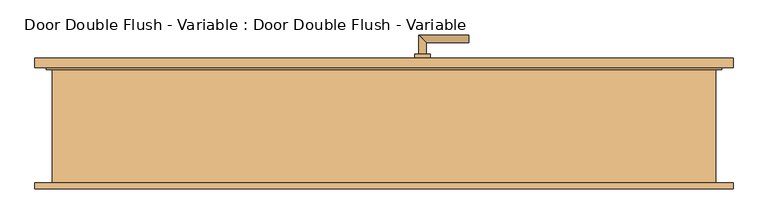
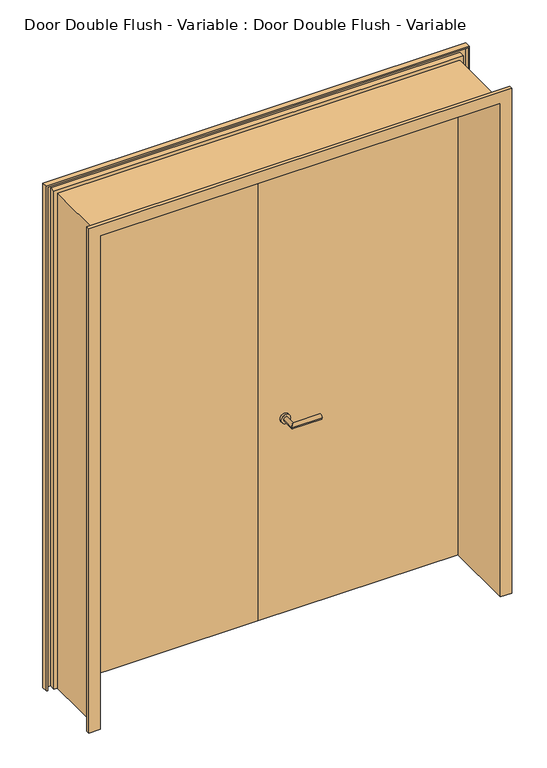
"""IFC4 building model written with IfcOpenShell, lengths in millimetres: door geometry, Door Double Flush - Variable : Door Double Flush - Variable."""

import ifcopenshell
import ifcopenshell.guid

model = None  # the IFC model being written
_history = None  # IfcOwnerHistory: only IFC2X3 demands one
_inside = {}  # id of a spatial element -> (the spatial element, [elements in it])
_under = {}  # id of a project, library or spatial element -> (it, [spatial elements below it])
_declared = {}  # id of a project -> (the project, [libraries it declares])
_typed = {}  # id of a type object -> (the type object, [elements of that type])
_made_of = {}  # id of a material, layer set ... -> (it, [elements and type objects made of it])


def new_model(schema):
    """Start an empty IFC model of exactly this schema.

    Asked for "IFC4X3", IfcOpenShell would pick the latest addendum, in which some entities
    have other attributes; the version numbers below select the first issue.
    IFC2X3 requires an IfcOwnerHistory on every rooted entity: one is made here for all.
    """
    global model, _history
    if schema == "IFC4X3":
        model = ifcopenshell.file(schema_version=(4, 3, 0, 0))
    else:
        model = ifcopenshell.file(schema=schema)
    _inside.clear()
    _under.clear()
    _declared.clear()
    _typed.clear()
    _made_of.clear()
    _history = None
    if model.schema == "IFC2X3":
        org = make("IfcOrganization", Name="unknown")
        user = make(
            "IfcPersonAndOrganization",
            ThePerson=make("IfcPerson", FamilyName="unknown"),
            TheOrganization=org,
        )
        app = make(
            "IfcApplication",
            ApplicationDeveloper=org,
            Version="unknown",
            ApplicationFullName="unknown",
            ApplicationIdentifier="unknown",
        )
        _history = make(
            "IfcOwnerHistory",
            OwningUser=user,
            OwningApplication=app,
            ChangeAction="ADDED",
            CreationDate=0,
        )
    return model


def make(cls, **values):
    """One entity of the class cls with the attributes given. An attribute that is None is left unset."""
    return model.create_entity(
        cls, **{name: value for name, value in values.items() if value is not None}
    )


def rooted(cls, **values):
    """An entity with a GlobalId (a new one), such as an element, a storey or a relation."""
    return make(cls, GlobalId=ifcopenshell.guid.new(), OwnerHistory=_history, **values)


def si_unit(unit_type, name, prefix=None):
    """IfcSIUnit, for example si_unit("LENGTHUNIT", "METRE", prefix="MILLI")."""
    return make("IfcSIUnit", UnitType=unit_type, Prefix=prefix, Name=name)


def assignment(units):
    """IfcUnitAssignment: the units of a project."""
    return None if units is None else make("IfcUnitAssignment", Units=units)


def point(xyz):
    """IfcCartesianPoint."""
    return None if xyz is None else make("IfcCartesianPoint", Coordinates=xyz)


def direction(xyz):
    """IfcDirection."""
    return None if xyz is None else make("IfcDirection", DirectionRatios=xyz)


def frame(location, z_axis=None, x_axis=None):
    """IfcAxis2Placement3D, a coordinate frame: its origin and axes. An axis left out is left unset."""
    return make(
        "IfcAxis2Placement3D",
        Location=point(location),
        Axis=direction(z_axis),
        RefDirection=direction(x_axis),
    )


def frame_2d(location, x_axis=None):
    """IfcAxis2Placement2D, a coordinate frame in the plane: its origin and x axis."""
    return make(
        "IfcAxis2Placement2D", Location=point(location), RefDirection=direction(x_axis)
    )


def origin():
    """The frame at (0, 0, 0) with its axes left unset."""
    return frame((0.0, 0.0, 0.0))


def place(relative_to, where):
    """IfcLocalPlacement: puts the frame where relative to a parent placement (None: the world)."""
    return make(
        "IfcLocalPlacement", PlacementRelTo=relative_to, RelativePlacement=where
    )


def context(
    kind, dimensions, precision=None, world=None, true_north=None, identifier=None
):
    """IfcGeometricRepresentationContext, for example the 3D "Model" context."""
    return make(
        "IfcGeometricRepresentationContext",
        ContextIdentifier=identifier,
        ContextType=kind,
        CoordinateSpaceDimension=dimensions,
        Precision=precision,
        WorldCoordinateSystem=world,
        TrueNorth=true_north,
    )


def project(units=None, contexts=None):
    """IfcProject with its units and contexts."""
    return rooted(
        "IfcProject",
        Name="project",
        RepresentationContexts=contexts,
        UnitsInContext=assignment(units),
    )


def spatial(cls, under=None, at=None, **own):
    """A site, building, storey or space (cls), placed at a placement, below another one or the project."""
    s = rooted(cls, ObjectPlacement=at, **own)
    if under is not None:
        _under.setdefault(under.id(), (under, []))[1].append(s)
    return s


def polyline(points):
    """IfcPolyline through the points."""
    return make("IfcPolyline", Points=[point(p) for p in points])


def circle_curve(where, radius):
    """IfcCircle in the frame where."""
    return make("IfcCircle", Position=where, Radius=radius)


def ellipse_curve(where, semi_axis1, semi_axis2):
    """IfcEllipse in the frame where."""
    return make(
        "IfcEllipse", Position=where, SemiAxis1=semi_axis1, SemiAxis2=semi_axis2
    )


def trimmed(basis, trim1, trim2, sense, master):
    """IfcTrimmedCurve: the piece of a basis curve between two trims."""
    return make(
        "IfcTrimmedCurve",
        BasisCurve=basis,
        Trim1=trim1,
        Trim2=trim2,
        SenseAgreement=sense,
        MasterRepresentation=master,
    )


def segment(curve, same_sense, transition):
    """IfcCompositeCurveSegment."""
    return make(
        "IfcCompositeCurveSegment",
        Transition=transition,
        SameSense=same_sense,
        ParentCurve=curve,
    )


def composite_curve(segments, self_intersect=None):
    """IfcCompositeCurve: segments joined end to end."""
    return make("IfcCompositeCurve", Segments=segments, SelfIntersect=self_intersect)


def outline(outer, holes=None, kind="AREA"):
    """IfcArbitraryClosedProfileDef: a profile drawn as a closed curve; with holes, ...WithVoids."""
    if holes is None:
        return make("IfcArbitraryClosedProfileDef", ProfileType=kind, OuterCurve=outer)
    return make(
        "IfcArbitraryProfileDefWithVoids",
        ProfileType=kind,
        OuterCurve=outer,
        InnerCurves=holes,
    )


def extrude(swept, where, along, depth):
    """IfcExtrudedAreaSolid: the profile swept, set in the frame where, extruded along a direction by depth."""
    return make(
        "IfcExtrudedAreaSolid",
        SweptArea=swept,
        Position=where,
        ExtrudedDirection=direction(along),
        Depth=depth,
    )


def faces_of(points, faces, orient=None, outer=None):
    """IfcFace entities. A face is a list of loops; a loop is a list of indices into points, from 0.

    orient and outer hold one flag for each loop. By default every Orientation is true, the
    first loop of a face is its IfcFaceOuterBound and the others are IfcFaceBound.
    """
    made = []
    for i, loops in enumerate(faces):
        bounds = []
        for j, loop in enumerate(loops):
            is_outer = j == 0 if outer is None else outer[i][j]
            bounds.append(
                make(
                    "IfcFaceOuterBound" if is_outer else "IfcFaceBound",
                    Bound=make("IfcPolyLoop", Polygon=[points[k] for k in loop]),
                    Orientation=True if orient is None else orient[i][j],
                )
            )
        made.append(make("IfcFace", Bounds=bounds))
    return made


def faceted_brep(points, faces, orient=None, outer=None, voids=None):
    """IfcFacetedBrep: a solid bounded by flat faces; with voids (closed shells), ...WithVoids."""
    shared = [point(p) for p in points]
    hull = make("IfcClosedShell", CfsFaces=faces_of(shared, faces, orient, outer))
    if voids is None:
        return make("IfcFacetedBrep", Outer=hull)
    return make(
        "IfcFacetedBrepWithVoids",
        Outer=hull,
        Voids=[
            make(cls, CfsFaces=faces_of(shared, fs, o, b)) for cls, fs, o, b in voids
        ],
    )


def shape(context_of_items, identifier, shape_type, items):
    """IfcShapeRepresentation: the items that make up one representation, for example the "Body"."""
    return make(
        "IfcShapeRepresentation",
        ContextOfItems=context_of_items,
        RepresentationIdentifier=identifier,
        RepresentationType=shape_type,
        Items=items,
    )


def source(mapping_origin, context_of_items, identifier, shape_type, items):
    """IfcRepresentationMap: a shape defined once, which mapped items show again and again."""
    return make(
        "IfcRepresentationMap",
        MappingOrigin=mapping_origin,
        MappedRepresentation=shape(context_of_items, identifier, shape_type, items),
    )


def transform(
    local_origin,
    x_axis=None,
    y_axis=None,
    z_axis=None,
    scale=None,
    scale2=None,
    scale3=None,
    uniform=True,
):
    """IfcCartesianTransformationOperator3D, or its non-uniform kind. x_axis, y_axis, z_axis: its Axis1, 2, 3."""
    if uniform:
        return make(
            "IfcCartesianTransformationOperator3D",
            Axis1=direction(x_axis),
            Axis2=direction(y_axis),
            LocalOrigin=point(local_origin),
            Scale=scale,
            Axis3=direction(z_axis),
        )
    return make(
        "IfcCartesianTransformationOperator3DnonUniform",
        Axis1=direction(x_axis),
        Axis2=direction(y_axis),
        LocalOrigin=point(local_origin),
        Scale=scale,
        Axis3=direction(z_axis),
        Scale2=scale2,
        Scale3=scale3,
    )


def mapped(mapping_source, mapping_target):
    """IfcMappedItem: shows the shape of a source again, moved by a transform."""
    return make(
        "IfcMappedItem", MappingSource=mapping_source, MappingTarget=mapping_target
    )


def made_of(thing, what):
    """Note that an element or type object is made of a material, layer set ...; save() writes the relation."""
    if what is not None:
        _made_of.setdefault(what.id(), (what, []))[1].append(thing)
    return thing


def element(
    cls,
    number,
    at=None,
    inside=None,
    cuts=None,
    type_object=None,
    material=None,
    context=None,
    identifier="Body",
    shape_type=None,
    held_by="IfcProductDefinitionShape",
    body=None,
    shapes=None,
    **own,
):
    """One element of the class cls, such as IfcWall. Its Tag is "e" and its number.

    at: its placement. inside: the storey or other place that contains it. cuts: it is an
    opening in that element (IfcRelVoidsElement). A single representation is given by context,
    identifier, shape_type and body (its items); several are given by shapes. held_by: the class
    of the entity that holds the representations. save() writes the other relations.
    """
    e = rooted(cls, Tag="e%d" % number, ObjectPlacement=at, **own)
    if body is not None:
        shapes = [shape(context, identifier, shape_type, body)]
    if shapes is not None:
        e.Representation = make(held_by, Representations=shapes)
    if inside is not None:
        _inside.setdefault(inside.id(), (inside, []))[1].append(e)
    if cuts is not None:
        rooted(
            "IfcRelVoidsElement", RelatingBuildingElement=cuts, RelatedOpeningElement=e
        )
    if type_object is not None:
        _typed.setdefault(type_object.id(), (type_object, []))[1].append(e)
    return made_of(e, material)


def aggregate(whole, parts):
    """IfcRelAggregates: a whole, such as a stair, and the parts it consists of."""
    return rooted("IfcRelAggregates", RelatingObject=whole, RelatedObjects=parts)


def save(model, path):
    """Write the relations noted so far, then the file.

    IfcRelAggregates (storeys below a building ...), IfcRelContainedInSpatialStructure (elements
    in a storey), IfcRelDefinesByType, IfcRelAssociatesMaterial and IfcRelDeclares: one each for
    every whole, place, type object, material and project.
    """
    for whole, parts in _under.values():
        aggregate(whole, parts)
    for where, things in _inside.values():
        rooted(
            "IfcRelContainedInSpatialStructure",
            RelatedElements=things,
            RelatingStructure=where,
        )
    for kind, things in _typed.values():
        rooted("IfcRelDefinesByType", RelatedObjects=things, RelatingType=kind)
    for what, things in _made_of.values():
        rooted("IfcRelAssociatesMaterial", RelatedObjects=things, RelatingMaterial=what)
    for by, libraries in _declared.values():
        rooted("IfcRelDeclares", RelatingContext=by, RelatedDefinitions=libraries)
    model.write(path)


def plane_surface(at):
    """IfcPlane: the flat surface through the origin of the frame at, square to its z axis."""
    return make("IfcPlane", Position=at)


def cylinder_surface(at, radius):
    """IfcCylindricalSurface: all points at the distance radius from the z axis of the frame at."""
    return make("IfcCylindricalSurface", Position=at, Radius=radius)


def advanced_brep(points, edges, surfaces, faces):
    """IfcAdvancedBrep: a solid bounded by faces that lie on surfaces and meet in shared edges.

    An edge is (start, end): straight between two places in points (the first is 0);
    or (start, end, curve); or (start, end, curve, False) where it runs against its curve.
    A face is (place in surfaces, loops), or (place, loops, False) where it looks against
    its surface's normal. A loop lists edges by number (the first is 1), with a minus sign
    where the edge is run from its end to its start. The first loop is the outer one.
    """
    corners = [point(p) for p in points]
    vertices = [make("IfcVertexPoint", VertexGeometry=c) for c in corners]
    made = []
    for start, end, *more in edges:
        made.append(
            make(
                "IfcEdgeCurve",
                EdgeStart=vertices[start],
                EdgeEnd=vertices[end],
                EdgeGeometry=more[0] if more else make("IfcPolyline", Points=[corners[start], corners[end]]),
                SameSense=more[1] if len(more) > 1 else True,
            )
        )
    hull = []
    for where, loops, *sense in faces:
        bounds = []
        for j, loop in enumerate(loops):
            ring = [make("IfcOrientedEdge", EdgeElement=made[abs(k) - 1], Orientation=k > 0) for k in loop]
            bounds.append(
                make(
                    "IfcFaceOuterBound" if j == 0 else "IfcFaceBound",
                    Bound=make("IfcEdgeLoop", EdgeList=ring),
                    Orientation=True,
                )
            )
        hull.append(make("IfcAdvancedFace", Bounds=bounds, FaceSurface=surfaces[where], SameSense=sense[0] if sense else True))
    return make("IfcAdvancedBrep", Outer=make("IfcClosedShell", CfsFaces=hull))


def door_double_flush_variable_door_double_flush_variable_ac6c3b87(model_context):
    return source(origin(), model_context, "Body", "SolidModel", [
        advanced_brep(
        [(90.0, 139.4346141, 1000.0), (110.0, 139.4346141, 1000.0), (90.0, 69.4346141, 1000.0), (110.0, 89.4346141, 1000.0), (220.0, 69.4346141, 1000.0), (220.0, 89.4346141, 1000.0)],
        [
            (0, 1, circle_curve(frame((100.0, 139.4346141, 1000.0), z_axis=(0.0, 1.0, 0.0), x_axis=(1.0, 0.0, 0.0)), 10.0)),
            (1, 0, circle_curve(frame((100.0, 139.4346141, 1000.0), z_axis=(0.0, 1.0, 0.0), x_axis=(1.0, 0.0, 0.0)), 10.0)),
            (0, 2),
            (2, 3, ellipse_curve(frame((100.0, 79.4346141, 1000.0), z_axis=(-0.7071067811865385, 0.7071067811865565, 0.0), x_axis=(0.7071067811865563, 0.7071067811865386, 0.0)), 14.1421356, 10.0)),
            (3, 1),
            (3, 2, ellipse_curve(frame((100.0, 79.4346141, 1000.0), z_axis=(-0.7071067811865385, 0.7071067811865565, 0.0), x_axis=(0.7071067811865563, 0.7071067811865386, 0.0)), 14.1421356, 10.0)),
            (4, 5, circle_curve(frame((220.0, 79.4346141, 1000.0), z_axis=(1.0, 0.0, 0.0), x_axis=(0.0, 1.0, 0.0)), 10.0)),
            (5, 4, circle_curve(frame((220.0, 79.4346141, 1000.0), z_axis=(1.0, 0.0, 0.0), x_axis=(0.0, 1.0, 0.0)), 10.0)),
            (2, 4),
            (5, 3),
        ],
        [
            plane_surface(frame((100.0, 139.4346141, -287.7526403), z_axis=(0.0, 1.0, 0.0), x_axis=(0.0, 0.0, 1.0))),
            cylinder_surface(frame((100.0, 139.4346141, 1000.0), z_axis=(0.0, 1.0, 0.0), x_axis=(1.0, 0.0, 0.0)), 10.0),
            plane_surface(frame((220.0, 79.4346141, -287.7526403), z_axis=(1.0, 0.0, 0.0), x_axis=(0.0, 0.0, 1.0))),
            cylinder_surface(frame((100.0, 79.4346141, 1000.0), z_axis=(-1.0, 0.0, 0.0), x_axis=(0.0, 1.0, 0.0)), 10.0),
        ],
        [
            (0, [[1, 2]]),
            (1, [[-1, 3, 4, 5]]),
            (1, [[-2, -5, 6, -3]]),
            (2, [[7, 8]]),
            (3, [[-4, 9, -8, 10]]),
            (3, [[-6, -10, -7, -9]]),
        ],
    ),
        advanced_brep(
        [(110.0, 199.4346141, 1000.0), (90.0, 199.4346141, 1000.0), (110.0, 229.4346141, 1000.0), (90.0, 249.4346141, 1000.0), (220.0, 229.4346141, 1000.0), (220.0, 249.4346141, 1000.0)],
        [
            (0, 1, circle_curve(frame((100.0, 199.4346141, 1000.0), z_axis=(0.0, -1.0, 0.0), x_axis=(-1.0, 0.0, 0.0)), 10.0)),
            (1, 0, circle_curve(frame((100.0, 199.4346141, 1000.0), z_axis=(0.0, -1.0, 0.0), x_axis=(-1.0, 0.0, 0.0)), 10.0)),
            (0, 2),
            (2, 3, ellipse_curve(frame((100.0, 239.4346141, 1000.0), z_axis=(-0.7071067811865475, -0.7071067811865475, 0.0), x_axis=(0.7071067811865474, -0.7071067811865476, 0.0)), 14.1421356, 10.0)),
            (3, 1),
            (3, 2, ellipse_curve(frame((100.0, 239.4346141, 1000.0), z_axis=(-0.7071067811865475, -0.7071067811865475, 0.0), x_axis=(0.7071067811865474, -0.7071067811865476, 0.0)), 14.1421356, 10.0)),
            (4, 5, circle_curve(frame((220.0, 239.4346141, 1000.0), z_axis=(1.0, 0.0, 0.0), x_axis=(0.0, 1.0, 0.0)), 10.0)),
            (5, 4, circle_curve(frame((220.0, 239.4346141, 1000.0), z_axis=(1.0, 0.0, 0.0), x_axis=(0.0, 1.0, 0.0)), 10.0)),
            (2, 4),
            (5, 3),
        ],
        [
            plane_surface(frame((100.0, 199.4346141, -287.7526403), z_axis=(0.0, -1.0, 0.0), x_axis=(0.0, 0.0, 1.0))),
            cylinder_surface(frame((100.0, 199.4346141, 1000.0), z_axis=(0.0, -1.0, 0.0), x_axis=(-1.0, 0.0, 0.0)), 10.0),
            plane_surface(frame((220.0, 239.4346141, -287.7526403), z_axis=(1.0, 0.0, 0.0), x_axis=(0.0, 0.0, 1.0))),
            cylinder_surface(frame((100.0, 239.4346141, 1000.0), z_axis=(-1.0, 0.0, 0.0), x_axis=(0.0, 1.0, 0.0)), 10.0),
        ],
        [
            (0, [[1, 2]]),
            (1, [[-1, 3, 4, 5]]),
            (1, [[-2, -5, 6, -3]]),
            (2, [[7, 8]]),
            (3, [[-4, 9, -8, 10]]),
            (3, [[-6, -10, -7, -9]]),
        ],
    ),
        extrude(outline(composite_curve([segment(trimmed(circle_curve(frame_2d((1000.0, 100.0)), 20.0), [point((1000.0, 80.0))], [point((1000.0, 120.0))], False, "CARTESIAN"), True, "CONTINUOUS"), segment(trimmed(circle_curve(frame_2d((1000.0, 100.0)), 20.0), [point((1000.0, 120.0))], [point((1000.0, 80.0))], False, "CARTESIAN"), True, "CONTINUOUS")], self_intersect=False)), frame((0.0, 129.4346141, 0.0), z_axis=(0.0, 1.0, 0.0), x_axis=(0.0, 0.0, 1.0)), (0.0, 0.0, 1.0), 10.0),
        extrude(outline(composite_curve([segment(trimmed(circle_curve(frame_2d((1000.0, 100.0)), 20.0), [point((1000.0, 80.0))], [point((1000.0, 120.0))], False, "CARTESIAN"), True, "CONTINUOUS"), segment(trimmed(circle_curve(frame_2d((1000.0, 100.0)), 20.0), [point((1000.0, 120.0))], [point((1000.0, 80.0))], False, "CARTESIAN"), True, "CONTINUOUS")], self_intersect=False)), frame((0.0, 189.4346141, 0.0), z_axis=(0.0, 1.0, 0.0), x_axis=(0.0, 0.0, 1.0)), (0.0, 0.0, 1.0), 10.0),
        extrude(outline(polyline([(0.0, 164.4346141), (-871.25, 164.4346141), (-871.25, 189.4346141), (0.0, 189.4346141), (0.0, 164.4346141)])), frame((0.0, 0.0, 100.0), z_axis=(0.0, 0.0, 1.0), x_axis=(1.0, 0.0, 0.0)), (0.0, 0.0, 1.0), 2250.0),
        extrude(outline(polyline([(871.25, 164.4346141), (0.0, 164.4346141), (0.0, 189.4346141), (871.25, 189.4346141), (871.25, 164.4346141)])), frame((0.0, 0.0, 100.0), z_axis=(0.0, 0.0, 1.0), x_axis=(1.0, 0.0, 0.0)), (0.0, 0.0, 1.0), 2250.0),
        faceted_brep([(905.75, -150.5653859, 100.0), (856.25, -150.5653859, 100.0), (856.25, 164.4346141, 100.0), (871.25, 164.4346141, 100.0), (871.25, 189.4346141, 100.0), (905.75, 189.4346141, 100.0), (905.75, 164.4346141, 100.0), (900.75, 164.4346141, 100.0), (900.75, 184.4346141, 100.0), (876.25, 184.4346141, 100.0), (876.25, 159.4346141, 100.0), (861.25, 159.4346141, 100.0), (861.25, -145.5653859, 100.0), (900.75, -145.5653859, 100.0), (900.75, -135.5653859, 100.0), (905.75, -135.5653859, 100.0), (905.75, -150.5653859, 2384.5), (-905.75, -150.5653859, 2384.5), (-905.75, -150.5653859, 100.0), (-856.25, -150.5653859, 100.0), (-856.25, -150.5653859, 2335.0), (856.25, -150.5653859, 2335.0), (856.25, 164.4346141, 2335.0), (-856.25, 164.4346141, 2335.0), (-856.25, 164.4346141, 100.0), (-871.25, 164.4346141, 100.0), (-871.25, 164.4346141, 2350.0), (871.25, 164.4346141, 2350.0), (871.25, 189.4346141, 2350.0), (-871.25, 189.4346141, 2350.0), (-871.25, 189.4346141, 100.0), (-905.75, 189.4346141, 100.0), (-905.75, 189.4346141, 2384.5), (905.75, 189.4346141, 2384.5), (905.75, 164.4346141, 2384.5), (-905.75, 164.4346141, 2384.5), (-905.75, 164.4346141, 100.0), (-900.75, 164.4346141, 100.0), (-900.75, 164.4346141, 2379.5), (900.75, 164.4346141, 2379.5), (900.75, 184.4346141, 2379.5), (-900.75, 184.4346141, 2379.5), (-900.75, 184.4346141, 100.0), (-876.25, 184.4346141, 100.0), (-876.25, 184.4346141, 2355.0), (876.25, 184.4346141, 2355.0), (876.25, 159.4346141, 2355.0), (-876.25, 159.4346141, 2355.0), (-876.25, 159.4346141, 100.0), (-861.25, 159.4346141, 100.0), (-861.25, 159.4346141, 2340.0), (861.25, 159.4346141, 2340.0), (861.25, -145.5653859, 2340.0), (-861.25, -145.5653859, 2340.0), (-861.25, -145.5653859, 100.0), (-900.75, -145.5653859, 100.0), (-900.75, -145.5653859, 2379.5), (900.75, -145.5653859, 2379.5), (900.75, -135.5653859, 2379.5), (-900.75, -135.5653859, 2379.5), (-900.75, -135.5653859, 100.0), (-905.75, -135.5653859, 100.0), (-905.75, -135.5653859, 2384.5), (905.75, -135.5653859, 2384.5)], [[[0, 1, 2, 3, 4, 5, 6, 7, 8, 9, 10, 11, 12, 13, 14, 15]], [[1, 0, 16, 17, 18, 19, 20, 21]], [[2, 1, 21, 22]], [[3, 2, 22, 23, 24, 25, 26, 27]], [[4, 3, 27, 28]], [[5, 4, 28, 29, 30, 31, 32, 33]], [[6, 5, 33, 34]], [[7, 6, 34, 35, 36, 37, 38, 39]], [[8, 7, 39, 40]], [[9, 8, 40, 41, 42, 43, 44, 45]], [[10, 9, 45, 46]], [[11, 10, 46, 47, 48, 49, 50, 51]], [[12, 11, 51, 52]], [[13, 12, 52, 53, 54, 55, 56, 57]], [[14, 13, 57, 58]], [[15, 14, 58, 59, 60, 61, 62, 63]], [[0, 15, 63, 16]], [[17, 62, 61, 18]], [[18, 61, 60, 55, 54, 49, 48, 43, 42, 37, 36, 31, 30, 25, 24, 19]], [[23, 20, 19, 24]], [[29, 26, 25, 30]], [[35, 32, 31, 36]], [[41, 38, 37, 42]], [[47, 44, 43, 48]], [[53, 50, 49, 54]], [[59, 56, 55, 60]], [[22, 21, 20, 23]], [[28, 27, 26, 29]], [[34, 33, 32, 35]], [[40, 39, 38, 41]], [[46, 45, 44, 47]], [[52, 51, 50, 53]], [[58, 57, 56, 59]], [[16, 63, 62, 17]]]),
    ])


if __name__ == "__main__":
    model = new_model("IFC4")
    model_context = context("Model", 3, world=origin())
    ifc_project = project(units=[si_unit("LENGTHUNIT", "METRE", prefix="MILLI")], contexts=[model_context])
    site = spatial("IfcSite", under=ifc_project)
    building = spatial("IfcBuilding", under=site)
    placement = place(None, origin())
    door_double_flush_variable_door_double_flush_variable_shape = door_double_flush_variable_door_double_flush_variable_ac6c3b87(model_context)
    element("IfcDoor", 1, ObjectType="Door Double Flush - Variable : Door Double Flush - Variable", at=placement, inside=building, context=model_context, shape_type="MappedRepresentation", body=[
        mapped(door_double_flush_variable_door_double_flush_variable_shape, transform((0.0, 0.0, 0.0), x_axis=(1.0, 0.0, 0.0), y_axis=(0.0, 1.0, 0.0), z_axis=(0.0, 0.0, 1.0))),
    ])
    save(model, "model.ifc")

# Revit data of these elements
# Type "Door Double Flush - Variable : Door Double Flush - Variable"
#   Type Mark = "33"
#   Operation = "DoubleDoorSingleSwing"
#   Keynote = "16.03"
#   Rough Width [instance default] = 2.010 m
#   Rough Height [instance default] = 2.360 m
#   Doorhandle Height = 0.900 m
#   Height [instance default] = 2.260 m
#   Sill Height [instance default] = 0.100 m
#   Width [instance default] = 2.010 m
#   Visibility [instance default] = yes
#   Doorhandle choose [instance default] = element 138974
#   Doorhandle [instance default] = Metal _ Chrome
#   Door [instance default] = Door - Wood
#   Frame [instance default] = Door - Wood
#   Function = (empty or 0)
#   Wall Closure = (empty or 0)
#   Assembly Code = ""
# Element 1 (IfcDoor, "Door Double Flush - Variable : Door Double Flush - Variable")
#   Rough Width = 1.7625 m
#   Width = 1.7625 m
#   Materials on its faces: "Door - Wood", "Metal _ Chrome"
# Materials
#   "Metal _ Chrome": class "Metall", colour RGB 247 247 247, transparency 0
#   "Door - Wood": class "Unassigned", colour RGB 114 94 79, transparency 0
